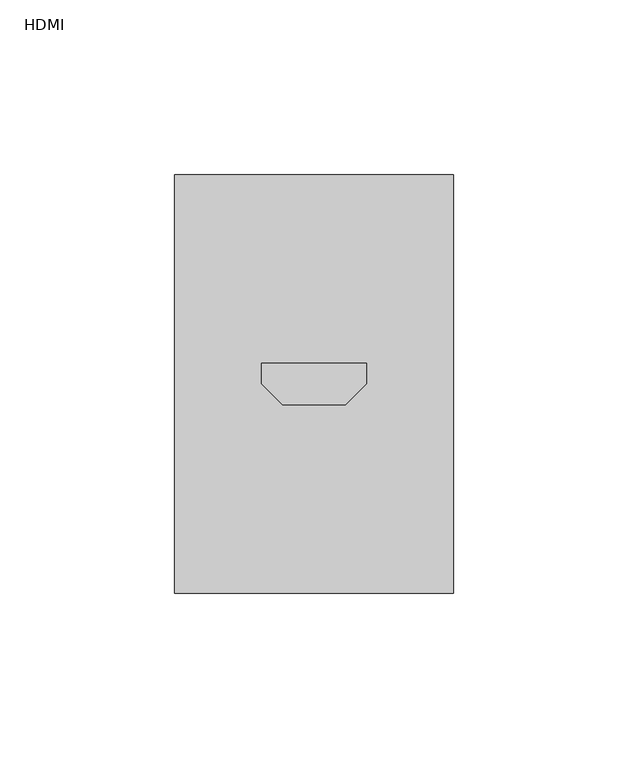
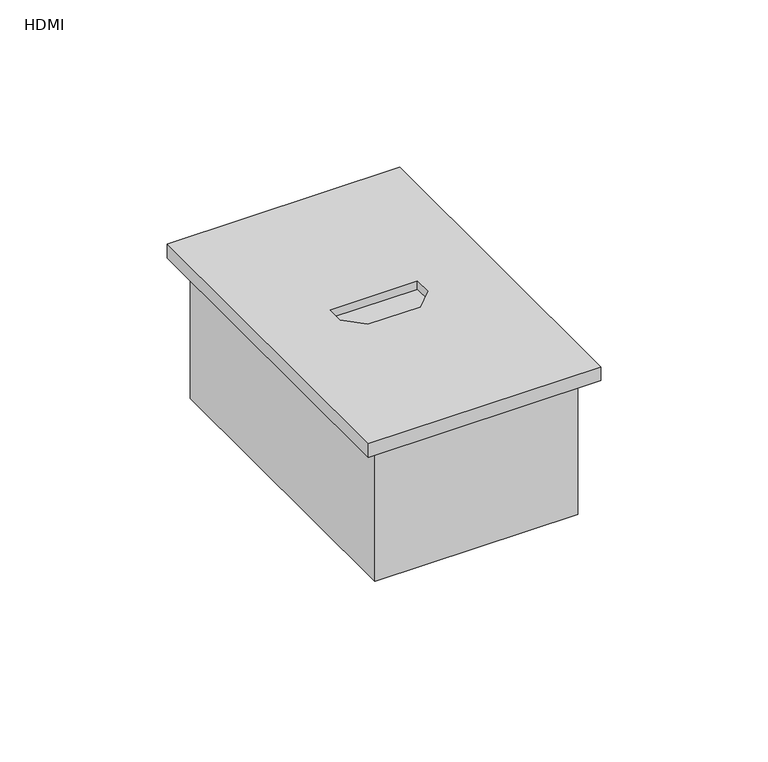
"""IFC4 building model written with IfcOpenShell, lengths in millimetres: proxy geometry, CAIXA VERTICE V7 : HDMI."""

from ifc_helpers import new_model, si_unit, origin, place, context, project, spatial, faceted_brep, source, transform, mapped, element, save


def hdmi_3e620413(model_context):
    return source(origin(), model_context, "Body", "Brep", [
        faceted_brep([(33.0, -1047.0, -48.0), (-33.0, -1047.0, -48.0), (-33.0, -1153.0, -48.0), (33.0, -1153.0, -48.0), (35.0, -1155.0, -50.0), (-35.0, -1155.0, -50.0), (-35.0, -1045.0, -50.0), (35.0, -1045.0, -50.0), (35.0, -1155.0, 0.0), (-35.0, -1155.0, 0.0), (-35.0, -1045.0, 0.0), (35.0, -1045.0, 0.0), (33.0, -1153.0, 0.0), (-33.0, -1153.0, 0.0), (-33.0, -1047.0, 0.0), (33.0, -1047.0, 0.0)], [[[0, 1, 2, 3]], [[4, 5, 6, 7]], [[4, 8, 9, 5]], [[9, 10, 6, 5]], [[10, 11, 7, 6]], [[11, 8, 4, 7]], [[8, 11, 10, 9], [12, 13, 14, 15]], [[15, 0, 3, 12]], [[14, 1, 0, 15]], [[13, 2, 1, 14]], [[12, 3, 2, 13]]]),
        faceted_brep([(40.0, -1160.0, 5.0), (40.0, -1040.0, 5.0), (-40.0, -1040.0, 5.0), (-40.0, -1160.0, 5.0), (-15.0, -1094.0, 5.0), (15.0, -1094.0, 5.0), (15.0, -1100.0, 5.0), (9.0, -1106.0, 5.0), (-9.0, -1106.0, 5.0), (-15.0, -1100.0, 5.0), (-40.0, -1160.0, 0.0), (-40.0, -1040.0, 0.0), (40.0, -1040.0, 0.0), (40.0, -1160.0, 0.0), (-15.0, -1094.0, 2.0), (-15.0, -1100.0, 2.0), (-9.0, -1106.0, 2.0), (9.0, -1106.0, 2.0), (15.0, -1100.0, 2.0), (15.0, -1094.0, 2.0)], [[[0, 1, 2, 3], [4, 5, 6, 7, 8, 9]], [[10, 11, 12, 13]], [[3, 10, 13, 0]], [[2, 11, 10, 3]], [[1, 12, 11, 2]], [[0, 13, 12, 1]], [[14, 4, 9, 15]], [[15, 9, 8, 16]], [[17, 7, 6, 18]], [[17, 18, 19, 14, 15, 16]], [[16, 8, 7, 17]], [[18, 6, 5, 19]], [[19, 5, 4, 14]]]),
    ])


if __name__ == "__main__":
    model = new_model("IFC4")
    model_context = context("Model", 3, world=origin())
    ifc_project = project(units=[si_unit("LENGTHUNIT", "METRE", prefix="MILLI")], contexts=[model_context])
    site = spatial("IfcSite", under=ifc_project)
    building = spatial("IfcBuilding", under=site)
    placement = place(None, origin())
    hdmi_shape = hdmi_3e620413(model_context)
    element("IfcBuildingElementProxy", 1, Name="CAIXA VERTICE V7 : HDMI", ObjectType="CAIXA VERTICE V7 : HDMI", at=placement, inside=building, context=model_context, shape_type="MappedRepresentation", body=[
        mapped(hdmi_shape, transform((0.0, 0.0, 0.0), x_axis=(1.0, 0.0, 0.0), y_axis=(0.0, 1.0, 0.0), z_axis=(0.0, 0.0, 1.0))),
    ])
    save(model, "model.ifc")

# Revit data of these elements
# Type "CAIXA VERTICE V7 : HDMI"
#   URL = "www.facebook.com/verticetreinamentos"
#   SEÇÃO [instance default] = ""
#   Rotação [instance default] = 0.00°
#   LARGURA DA TAMPA = 0.08 m
#   BORDA = 0.01 m
#   ALTURA DE INSTALAÇÃO [instance default] = 1.10 m
#   Distância Anotação [instance default] = 0.0015 m
#   ALTURA DA TAMPA = 0.12 m
#   Vertical [instance default] = yes
#   VER SEÇÃO [instance default] = yes
#   SHADE ESQ [instance default] = no
#   SHADE DIR [instance default] = yes
#   HORIZONTAL [instance default] = no
#   ANDAR COM A LEGENDA [instance default] = 0
#   Material Tampa [instance default] = Plástico, branco opaco
#   Caixa = element 1798549
#   Anotação = element 1798548
#   Default Elevation = 0
# Element 1 (IfcBuildingElementProxy, "CAIXA VERTICE V7 : HDMI")
#   VER SEÇÃO = no
#   Materials on its faces: "Plástico, branco opaco"
# Materials
#   "Plástico, branco opaco": class "Plástico", colour RGB 120 120 120, transparency 0, Description = "Plastic, generic, opaque white", Cost = 0
